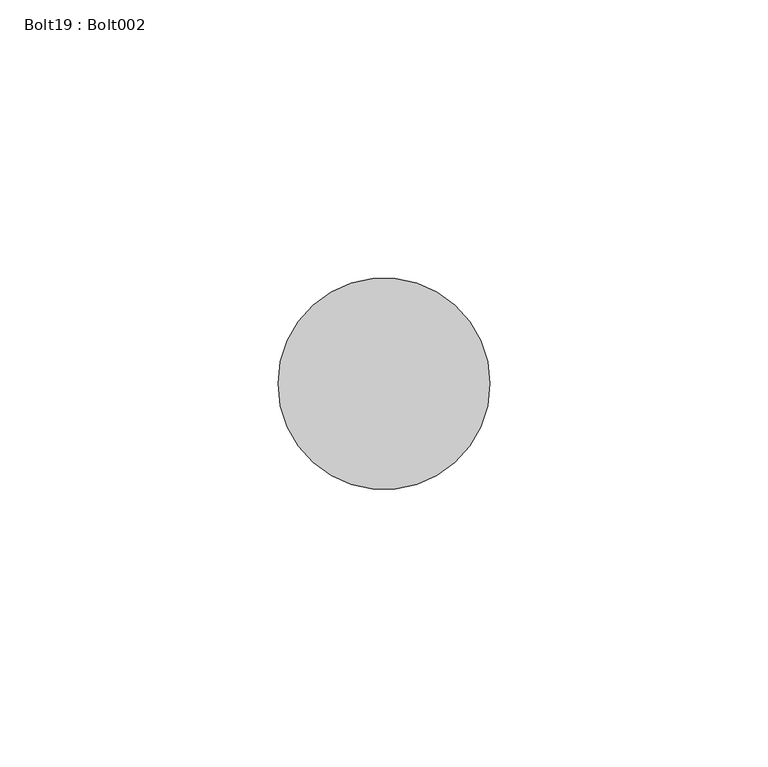
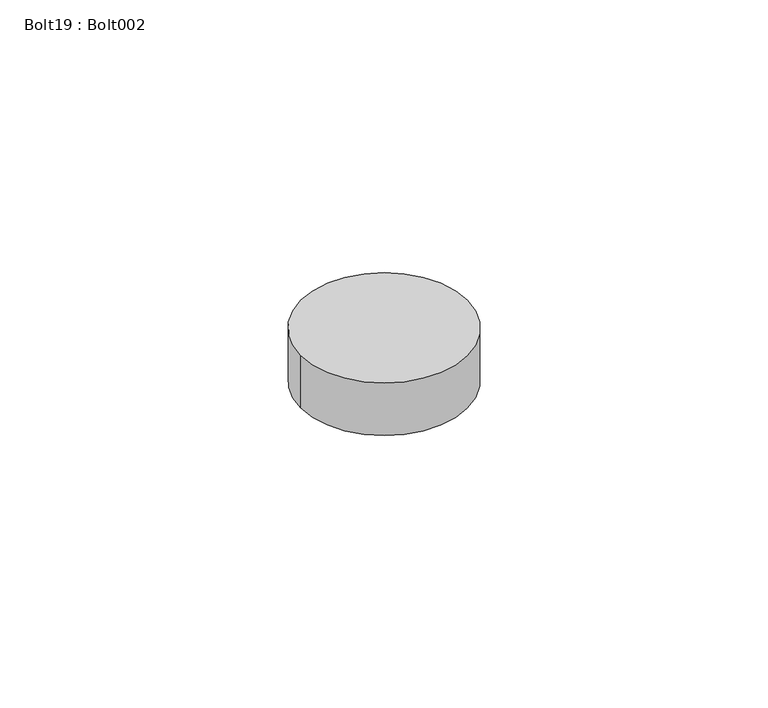
"""IFC4 building model written with IfcOpenShell, lengths in millimetres: proxy geometry, Bolt19 : Bolt002."""

from ifc_helpers import new_model, si_unit, point, frame, frame_2d, origin, place, context, project, spatial, circle_curve, trimmed, segment, composite_curve, outline, extrude, source, transform, mapped, element, save


def bolt19_bolt002_b789c14b(model_context):
    return source(origin(), model_context, "Body", "SweptSolid", [
        extrude(outline(composite_curve([segment(trimmed(circle_curve(frame_2d((7415.2612305, -1781.8449707)), 19.05), [point((7396.2112305, -1781.8449707))], [point((7434.3112305, -1781.8449707))], False, "CARTESIAN"), True, "CONTINUOUS"), segment(trimmed(circle_curve(frame_2d((7415.2612305, -1781.8449707)), 19.05), [point((7434.3112305, -1781.8449707))], [point((7396.2112305, -1781.8449707))], False, "CARTESIAN"), True, "CONTINUOUS")], self_intersect=False)), frame((0.0, 0.0, 40112.696), z_axis=(0.0, 0.0, 1.0), x_axis=(1.0, 0.0, 0.0)), (0.0, 0.0, 1.0), 12.7),
    ])


if __name__ == "__main__":
    model = new_model("IFC4")
    model_context = context("Model", 3, world=origin())
    ifc_project = project(units=[si_unit("LENGTHUNIT", "METRE", prefix="MILLI")], contexts=[model_context])
    site = spatial("IfcSite", under=ifc_project)
    building = spatial("IfcBuilding", under=site)
    placement = place(None, origin())
    bolt19_bolt002_shape = bolt19_bolt002_b789c14b(model_context)
    element("IfcBuildingElementProxy", 1, Name="Bolt19 : Bolt002", ObjectType="Bolt19 : Bolt002", at=placement, inside=building, context=model_context, shape_type="MappedRepresentation", body=[
        mapped(bolt19_bolt002_shape, transform((0.0, 0.0, 0.0), x_axis=(1.0, 0.0, 0.0), y_axis=(0.0, 1.0, 0.0), z_axis=(0.0, 0.0, 1.0))),
    ])
    save(model, "model.ifc")

# Revit data of these elements
# Type "Bolt19 : Bolt002"
#   NameOverride = "Bolt002"
# Element 1 (IfcBuildingElementProxy, "Bolt19 : Bolt002")
#   Materials on its faces: "BOLTS CONCEALED BY FLOOR FINISH"
# Materials
#   "BOLTS CONCEALED BY FLOOR FINISH": class "Unassigned", colour RGB 128 128 128, transparency 0
